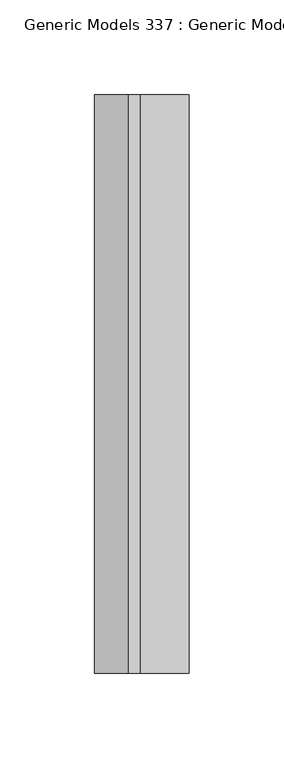
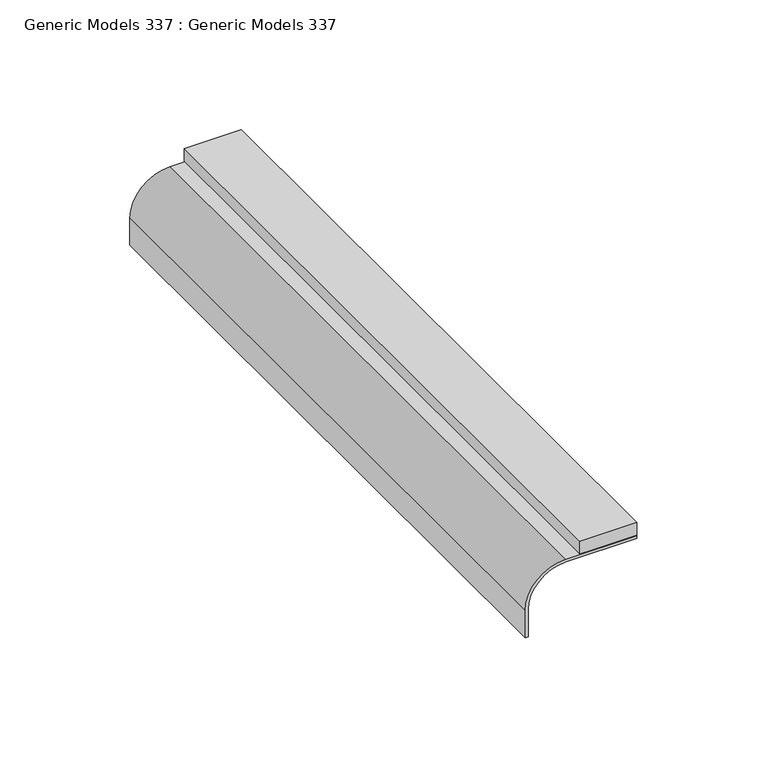
"""IFC4 building model written with IfcOpenShell, lengths in millimetres: proxy geometry, Generic Models 337 : Generic Models 337."""

from ifc_helpers import new_model, si_unit, point, frame, frame_2d, origin, place, context, project, spatial, polyline, circle_curve, trimmed, segment, composite_curve, outline, extrude, source, transform, mapped, element, save


def generic_models_337_generic_models_337_f6f16834(model_context):
    return source(origin(), model_context, "Body", "SweptSolid", [
        extrude(outline(composite_curve([segment(trimmed(circle_curve(frame_2d((126168.9854878, 8305.1784978)), 17.9605122), [point((126186.946, 8305.1784978))], [point((126168.9854878, 8287.2179855))], False, "CARTESIAN"), True, "CONTINUOUS"), segment(polyline([(126168.9854878, 8287.2179855), (126156.2854878, 8287.2179855), (126156.2854878, 8288.5078293), (126168.9854878, 8288.5078293)]), True, "CONTINUOUS"), segment(trimmed(circle_curve(frame_2d((126168.9854878, 8305.1784978)), 16.6706685), [point((126168.9854878, 8288.5078293))], [point((126185.6561563, 8305.1784978))], True, "CARTESIAN"), True, "CONTINUOUS"), segment(polyline([(126185.6561563, 8305.1784978), (126185.6561563, 8336.9284978), (126186.946, 8336.9284978), (126186.946, 8305.1784978)]), True, "CONTINUOUS")], self_intersect=False)), frame((0.0, -4109.6428838, 0.0), z_axis=(0.0, 1.0, 0.0), x_axis=(0.0, 0.0, 1.0)), (0.0, 0.0, 1.0), 304.8),
        extrude(outline(polyline([(8311.5284978, -3804.8428838), (8336.9284978, -3804.8428838), (8336.9284978, -4109.6428838), (8311.5284978, -4109.6428838), (8311.5284978, -3804.8428838)])), frame((0.0, 0.0, 126186.946), z_axis=(0.0, 0.0, 1.0), x_axis=(1.0, 0.0, 0.0)), (0.0, 0.0, 1.0), 6.35),
    ])


if __name__ == "__main__":
    model = new_model("IFC4")
    model_context = context("Model", 3, world=origin())
    ifc_project = project(units=[si_unit("LENGTHUNIT", "METRE", prefix="MILLI")], contexts=[model_context])
    site = spatial("IfcSite", under=ifc_project)
    building = spatial("IfcBuilding", under=site)
    placement = place(None, origin())
    generic_models_337_generic_models_337_shape = generic_models_337_generic_models_337_f6f16834(model_context)
    element("IfcBuildingElementProxy", 1, Name="Generic Models 337 : Generic Models 337", ObjectType="Generic Models 337 : Generic Models 337", at=placement, inside=building, context=model_context, shape_type="MappedRepresentation", body=[
        mapped(generic_models_337_generic_models_337_shape, transform((0.0, 0.0, 0.0), x_axis=(1.0, 0.0, 0.0), y_axis=(0.0, 1.0, 0.0), z_axis=(0.0, 0.0, 1.0))),
    ])
    save(model, "model.ifc")

# Revit data of these elements
# Element 1 (IfcBuildingElementProxy, "Generic Models 337 : Generic Models 337")
#   Materials on its faces: "_WEATHER STRIPPING"
# Materials
#   "_WEATHER STRIPPING": class "Generic", colour RGB 245 226 173, transparency 0, Cost = 0
